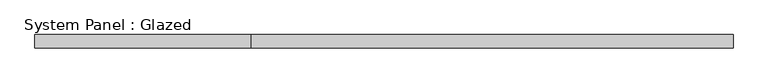
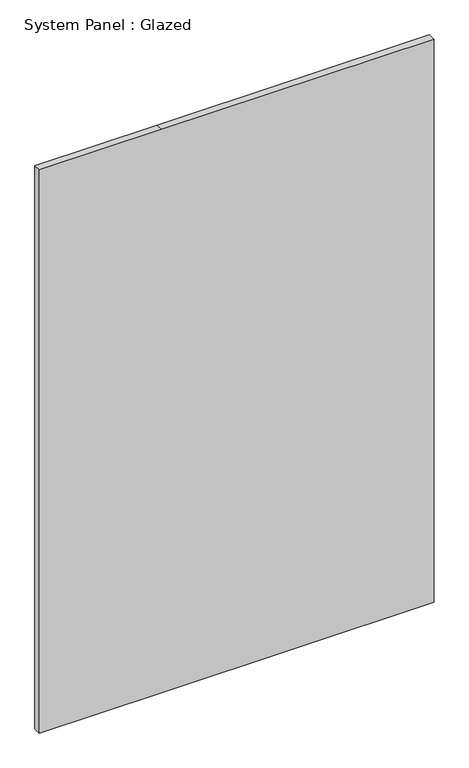
"""IFC4 building model written with IfcOpenShell, lengths in millimetres: plate geometry, System Panel : Glazed."""

from ifc_helpers import new_model, si_unit, frame, origin, place, context, project, spatial, polyline, outline, extrude, source, transform, mapped, element, save


def system_panel_glazed_bc4c4872(model_context):
    return source(origin(), model_context, "Body", "SweptSolid", [
        extrude(outline(polyline([(0.0, -676.275), (0.0, -257.175), (0.0, 676.275), (2038.35, 676.275), (2038.35, -257.175), (2038.35, -676.275), (0.0, -676.275)])), frame((0.0, -44.45, 0.0), z_axis=(0.0, 1.0, 0.0), x_axis=(0.0, 0.0, 1.0)), (0.0, 0.0, 1.0), 25.4),
    ])


if __name__ == "__main__":
    model = new_model("IFC4")
    model_context = context("Model", 3, world=origin())
    ifc_project = project(units=[si_unit("LENGTHUNIT", "METRE", prefix="MILLI")], contexts=[model_context])
    site = spatial("IfcSite", under=ifc_project)
    building = spatial("IfcBuilding", under=site)
    placement = place(None, origin())
    system_panel_glazed_shape = system_panel_glazed_bc4c4872(model_context)
    element("IfcPlate", 1, ObjectType="System Panel : Glazed", at=placement, inside=building, context=model_context, shape_type="MappedRepresentation", body=[
        mapped(system_panel_glazed_shape, transform((0.0, 0.0, 0.0), x_axis=(1.0, 0.0, 0.0), y_axis=(0.0, 1.0, 0.0), z_axis=(0.0, 0.0, 1.0))),
    ])
    save(model, "model.ifc")

# Revit data of these elements
# Type "System Panel : Glazed"
#   Construction Type Id = "GSP4R"
#   Analytic Construction = "1/8 in Pilkington single glazing"
#   Visual Light Transmittance = 0.9
#   Solar Heat Gain Coefficient = 0.86
#   Heat Transfer Coefficient (U) = 1.18115 BTU/(h·ft²·°F)
#   Define Thermal Properties by = 1
# Element 1 (IfcPlate, "System Panel : Glazed")
#   Materials on its faces: "Glass"
# Materials
#   "Glass": class "Glass", colour RGB 0 0 255, transparency 0.75, Description = "Soda Lime Glass", Cost = 0
